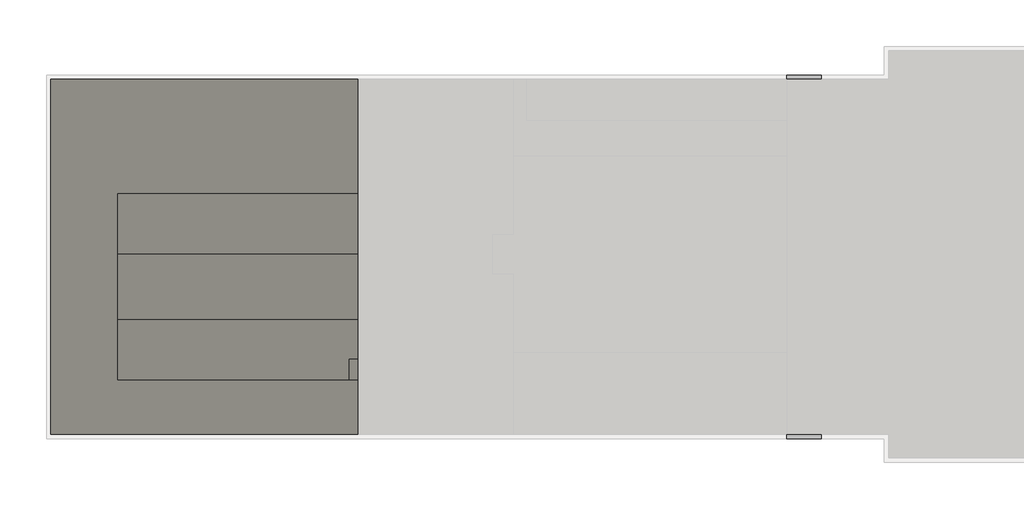
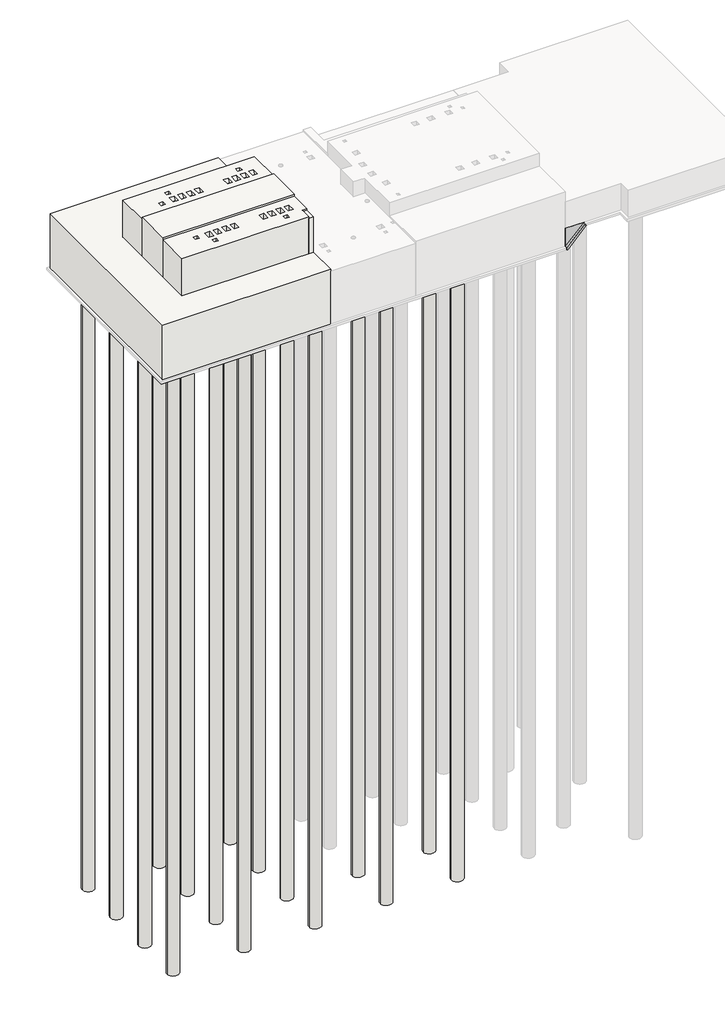
# One storey, part 1 of 2: 20 slabs, 2 proxies.
"""IFC4 building model written with IfcOpenShell, lengths in millimetres."""

from ifc_helpers import new_model, si_unit, point, frame, frame_2d, origin, place, context, project, spatial, polyline, circle_curve, trimmed, segment, composite_curve, outline, extrude, faceted_brep, element, save

model = new_model("IFC4")

# Units and contexts
model_context = context("Model", 3, world=origin())
ifc_project = project(units=[si_unit("LENGTHUNIT", "METRE", prefix="MILLI")], contexts=[model_context])

# Site, building, storey
site = spatial("IfcSite", under=ifc_project)
building = spatial("IfcBuilding", under=site)
storey = spatial("IfcBuildingStorey", under=building, Name="B.O.F", Elevation=2800.0)

# Proxies
placement = place(None, origin())
element("IfcBuildingElementProxy", 1, Name="H_SF_AR_S17_SOG Edge_800x800", ObjectType="H_SF_AR_S17_SOG Edge_800x800", at=placement, inside=storey, context=model_context, shape_type="SweptSolid", body=[
    extrude(outline(polyline([(3600.0, 17000.0), (2800.0, 17000.0), (3600.0, 17800.0), (3600.0, 17000.0)])), frame((0.0, -16046.5096992, 0.0), z_axis=(0.0, 1.0, 0.0), x_axis=(0.0, 0.0, 1.0)), (0.0, 0.0, 1.0), 8200.0),
])
element("IfcBuildingElementProxy", 2, Name="H_SF_AR_S18_Lean_T100_Slab Edge", ObjectType="H_SF_AR_S18_Lean_T100_Slab Edge", at=placement, inside=storey, context=model_context, shape_type="SweptSolid", body=[
    extrude(outline(polyline([(3600.0, 17800.0), (2800.0, 17000.0), (2700.0, 17000.0), (2700.0, 17041.4213562), (3500.0, 17841.4213562), (3500.0, 17800.0), (3600.0, 17800.0)])), frame((0.0, -16146.5096992, 0.0), z_axis=(0.0, 1.0, 0.0), x_axis=(0.0, 0.0, 1.0)), (0.0, 0.0, 1.0), 8400.0),
])

# Slabs
element("IfcSlab", 3, ObjectType="H_SF_AR_B01_EQ FDN_Bitumen_Mat T2440", at=placement, inside=storey, context=model_context, shape_type="Brep", body=[
    faceted_brep([(7095.0, -7846.5096992, 2800.0), (7095.0, -10486.5096992, 2800.0), (1545.0, -10486.5096992, 2800.0), (1545.0, -11886.5096992, 2800.0), (1545.0, -13386.5096992, 2800.0), (1545.0, -14786.5096992, 2800.0), (6895.0, -14786.5096992, 2800.0), (7095.0, -14786.5096992, 2800.0), (7095.0, -16046.5096992, 2800.0), (0.0, -16046.5096992, 2800.0), (0.0, -7846.5096992, 2800.0), (7095.0, -7846.5096992, 5240.0), (0.0, -7846.5096992, 5240.0), (0.0, -16046.5096992, 5240.0), (7095.0, -16046.5096992, 5240.0), (7095.0, -14786.5096992, 5240.0), (1545.0, -14786.5096992, 5240.0), (1545.0, -10486.5096992, 5240.0), (7095.0, -10486.5096992, 5240.0), (7095.0, -7846.5096992, 5150.0), (7095.0, -16046.5096992, 5150.0)], [[[0, 1, 2, 3, 4, 5, 6, 7, 8, 9, 10]], [[11, 12, 13, 14, 15, 16, 17, 18]], [[1, 0, 19, 11, 18]], [[2, 1, 18, 17]], [[5, 4, 3, 2, 17, 16]], [[7, 6, 5, 16, 15]], [[8, 7, 15, 14, 20]], [[9, 8, 20, 14, 13]], [[10, 9, 13, 12]], [[0, 10, 12, 11, 19]]]),
])
element("IfcSlab", 4, ObjectType="H_SF_AR_B01_EQ FDN_Bitumen_Mat T4188", at=placement, inside=storey, context=model_context, shape_type="Brep", body=[
    faceted_brep([(7095.0, -11886.5096992, 2800.0), (7095.0, -13386.5096992, 2800.0), (1545.0, -13386.5096992, 2800.0), (1545.0, -11886.5096992, 2800.0), (7095.0, -13386.5096992, 6988.0), (7095.0, -11886.5096992, 6988.0), (1545.0, -11886.5096992, 6988.0), (1545.0, -13386.5096992, 6988.0), (7095.0, -11886.5096992, 6893.0), (7095.0, -13386.5096992, 6893.0), (1545.0, -13386.5096992, 6893.0), (1545.0, -13386.5096992, 5240.0), (1545.0, -11886.5096992, 6893.0), (1545.0, -11886.5096992, 5240.0)], [[[0, 1, 2, 3]], [[4, 5, 6, 7]], [[1, 0, 8, 5, 4, 9]], [[2, 1, 9, 4, 7, 10, 11]], [[3, 2, 11, 10, 7, 6, 12, 13]], [[0, 3, 13, 12, 6, 5, 8]]]),
])
element("IfcSlab", 5, ObjectType="H_SF_AR_B01_EQ FDN_Bitumen_Mat T4093", at=placement, inside=storey, context=model_context, shape_type="Brep", body=[
    faceted_brep([(6895.0, -14786.5096992, 2800.0), (1545.0, -14786.5096992, 2800.0), (1545.0, -13386.5096992, 2800.0), (7095.0, -13386.5096992, 2800.0), (7095.0, -14316.5096992, 2800.0), (6895.0, -14316.5096992, 2800.0), (1545.0, -14786.5096992, 6893.0), (6895.0, -14786.5096992, 6893.0), (6895.0, -14316.5096992, 6893.0), (7095.0, -14316.5096992, 6893.0), (7095.0, -13386.5096992, 6893.0), (1545.0, -13386.5096992, 6893.0), (2590.0, -13801.5096992, 6893.0), (2760.0, -13801.5096992, 6893.0), (2760.0, -13971.5096992, 6893.0), (2590.0, -13971.5096992, 6893.0), (3110.0, -14286.5096992, 6893.0), (3280.0, -14286.5096992, 6893.0), (3280.0, -14456.5096992, 6893.0), (3110.0, -14456.5096992, 6893.0), (6110.0, -14286.5096992, 6893.0), (6280.0, -14286.5096992, 6893.0), (6280.0, -14456.5096992, 6893.0), (6110.0, -14456.5096992, 6893.0), (3095.0, -14086.5096992, 6893.0), (3095.0, -13786.5096992, 6893.0), (3295.0, -13786.5096992, 6893.0), (3295.0, -14086.5096992, 6893.0), (3445.0, -14086.5096992, 6893.0), (3445.0, -13786.5096992, 6893.0), (3645.0, -13786.5096992, 6893.0), (3645.0, -14086.5096992, 6893.0), (3808.0, -14086.5096992, 6893.0), (3808.0, -13786.5096992, 6893.0), (4008.0, -13786.5096992, 6893.0), (4008.0, -14086.5096992, 6893.0), (4158.0, -14086.5096992, 6893.0), (4158.0, -13786.5096992, 6893.0), (4358.0, -13786.5096992, 6893.0), (4358.0, -14086.5096992, 6893.0), (5382.0, -14086.5096992, 6893.0), (5382.0, -13786.5096992, 6893.0), (5582.0, -13786.5096992, 6893.0), (5582.0, -14086.5096992, 6893.0), (5732.0, -14086.5096992, 6893.0), (5732.0, -13786.5096992, 6893.0), (5932.0, -13786.5096992, 6893.0), (5932.0, -14086.5096992, 6893.0), (6095.0, -14086.5096992, 6893.0), (6095.0, -13786.5096992, 6893.0), (6295.0, -13786.5096992, 6893.0), (6295.0, -14086.5096992, 6893.0), (6445.0, -14086.5096992, 6893.0), (6445.0, -13786.5096992, 6893.0), (6645.0, -13786.5096992, 6893.0), (6645.0, -14086.5096992, 6893.0), (6895.0, -14786.5096992, 5240.0), (6895.0, -14786.5096992, 6833.0), (1545.0, -14786.5096992, 5240.0), (1545.0, -13386.5096992, 5240.0), (7095.0, -14316.5096992, 6833.0), (6895.0, -14316.5096992, 6833.0), (2760.0, -13801.5096992, 6592.9618634), (2590.0, -13801.5096992, 6592.9618634), (2590.0, -13971.5096992, 6592.9618634), (2760.0, -13971.5096992, 6592.9618634), (3280.0, -14286.5096992, 6592.9618634), (3110.0, -14286.5096992, 6592.9618634), (3110.0, -14456.5096992, 6592.9618634), (3280.0, -14456.5096992, 6592.9618634), (6280.0, -14286.5096992, 6592.9618634), (6110.0, -14286.5096992, 6592.9618634), (6110.0, -14456.5096992, 6592.9618634), (6280.0, -14456.5096992, 6592.9618634), (3095.0, -14011.509641, 6138.0), (3295.0, -14011.509641, 6138.0), (3295.0, -13761.5096992, 6138.0), (3095.0, -13761.5096992, 6138.0), (3095.0, -13986.5096992, 6743.0), (3295.0, -13986.5096877, 6743.0), (3445.0, -14011.509641, 6138.0), (3645.0, -14011.509641, 6138.0), (3645.0, -13761.5096992, 6138.0), (3445.0, -13761.5096992, 6138.0), (3445.0, -13986.5096992, 6743.0), (3645.0, -13986.5096877, 6743.0), (3808.0, -14011.509641, 6138.0), (4008.0, -14011.509641, 6138.0), (4008.0, -13761.5096992, 6138.0), (3808.0, -13761.5096992, 6138.0), (3808.0, -13986.5096992, 6743.0), (4008.0, -13986.5096877, 6743.0), (4158.0, -14011.509641, 6138.0), (4358.0, -14011.509641, 6138.0), (4358.0, -13761.5096992, 6138.0), (4158.0, -13761.5096992, 6138.0), (4158.0, -13986.5096992, 6743.0), (4358.0, -13986.5096877, 6743.0), (5382.0, -14011.509641, 6138.0), (5582.0, -14011.509641, 6138.0), (5582.0, -13761.5096992, 6138.0), (5382.0, -13761.5096992, 6138.0), (5382.0, -13986.5096992, 6743.0), (5582.0, -13986.5096877, 6743.0), (5732.0, -14011.509641, 6138.0), (5932.0, -14011.509641, 6138.0), (5932.0, -13761.5096992, 6138.0), (5732.0, -13761.5096992, 6138.0), (5732.0, -13986.5096992, 6743.0), (5932.0, -13986.5096877, 6743.0), (6095.0, -14011.509641, 6138.0), (6295.0, -14011.509641, 6138.0), (6295.0, -13761.5096992, 6138.0), (6095.0, -13761.5096992, 6138.0), (6095.0, -13986.5096992, 6743.0), (6295.0, -13986.5096877, 6743.0), (6445.0, -14011.509641, 6138.0), (6645.0, -14011.509641, 6138.0), (6645.0, -13761.5096992, 6138.0), (6445.0, -13761.5096992, 6138.0), (6445.0, -13986.5096992, 6743.0), (6645.0, -13986.5096877, 6743.0)], [[[0, 1, 2, 3, 4, 5]], [[6, 7, 8, 9, 10, 11], [12, 13, 14, 15], [16, 17, 18, 19], [20, 21, 22, 23], [24, 25, 26, 27], [28, 29, 30, 31], [32, 33, 34, 35], [36, 37, 38, 39], [40, 41, 42, 43], [44, 45, 46, 47], [48, 49, 50, 51], [52, 53, 54, 55]], [[1, 0, 56, 57, 7, 6, 58]], [[2, 1, 58, 6, 11, 59]], [[3, 2, 59, 11, 10]], [[4, 3, 10, 9, 60]], [[5, 4, 60, 9, 8, 61]], [[0, 5, 61, 8, 7, 57, 56]], [[62, 63, 64, 65]], [[63, 62, 13, 12]], [[64, 63, 12, 15]], [[65, 64, 15, 14]], [[62, 65, 14, 13]], [[66, 67, 68, 69]], [[67, 66, 17, 16]], [[68, 67, 16, 19]], [[69, 68, 19, 18]], [[66, 69, 18, 17]], [[70, 71, 72, 73]], [[71, 70, 21, 20]], [[72, 71, 20, 23]], [[73, 72, 23, 22]], [[70, 73, 22, 21]], [[74, 75, 76, 77]], [[74, 77, 25, 24, 78]], [[77, 76, 26, 25]], [[76, 75, 79, 27, 26]], [[75, 74, 78, 79]], [[78, 24, 27, 79]], [[80, 81, 82, 83]], [[80, 83, 29, 28, 84]], [[83, 82, 30, 29]], [[82, 81, 85, 31, 30]], [[81, 80, 84, 85]], [[86, 87, 88, 89]], [[86, 89, 33, 32, 90]], [[89, 88, 34, 33]], [[88, 87, 91, 35, 34]], [[87, 86, 90, 91]], [[92, 93, 94, 95]], [[92, 95, 37, 36, 96]], [[95, 94, 38, 37]], [[94, 93, 97, 39, 38]], [[93, 92, 96, 97]], [[98, 99, 100, 101]], [[98, 101, 41, 40, 102]], [[101, 100, 42, 41]], [[100, 99, 103, 43, 42]], [[99, 98, 102, 103]], [[104, 105, 106, 107]], [[104, 107, 45, 44, 108]], [[107, 106, 46, 45]], [[106, 105, 109, 47, 46]], [[105, 104, 108, 109]], [[110, 111, 112, 113]], [[110, 113, 49, 48, 114]], [[113, 112, 50, 49]], [[112, 111, 115, 51, 50]], [[111, 110, 114, 115]], [[116, 117, 118, 119]], [[116, 119, 53, 52, 120]], [[119, 118, 54, 53]], [[118, 117, 121, 55, 54]], [[117, 116, 120, 121]], [[84, 28, 31, 85]], [[90, 32, 35, 91]], [[96, 36, 39, 97]], [[102, 40, 43, 103]], [[108, 44, 47, 109]], [[114, 48, 51, 115]], [[120, 52, 55, 121]]]),
    faceted_brep([(7095.0, -10486.5096992, 2800.0), (7095.0, -11886.5096992, 2800.0), (1545.0, -11886.5096992, 2800.0), (1545.0, -10486.5096992, 2800.0), (7095.0, -11886.5096992, 6893.0), (7095.0, -10486.5096992, 6893.0), (1545.0, -10486.5096992, 6893.0), (1545.0, -11886.5096992, 6893.0), (2590.0, -11301.5096992, 6893.0), (2760.0, -11301.5096992, 6893.0), (2760.0, -11471.5096992, 6893.0), (2590.0, -11471.5096992, 6893.0), (3110.0, -10816.5096992, 6893.0), (3280.0, -10816.5096992, 6893.0), (3280.0, -10986.5096992, 6893.0), (3110.0, -10986.5096992, 6893.0), (6110.0, -10816.5096992, 6893.0), (6280.0, -10816.5096992, 6893.0), (6280.0, -10986.5096992, 6893.0), (6110.0, -10986.5096992, 6893.0), (3645.0, -11186.5096992, 6893.0), (3645.0, -11486.5096992, 6893.0), (3445.0, -11486.5096992, 6893.0), (3445.0, -11186.5096992, 6893.0), (3295.0, -11186.5096992, 6893.0), (3295.0, -11486.5096992, 6893.0), (3095.0, -11486.5096992, 6893.0), (3095.0, -11186.5096992, 6893.0), (4008.0, -11186.5096992, 6893.0), (4008.0, -11486.5096992, 6893.0), (3808.0, -11486.5096992, 6893.0), (3808.0, -11186.5096992, 6893.0), (4358.0, -11186.5096992, 6893.0), (4358.0, -11486.5096992, 6893.0), (4158.0, -11486.5096992, 6893.0), (4158.0, -11186.5096992, 6893.0), (5582.0, -11186.5096992, 6893.0), (5582.0, -11486.5096992, 6893.0), (5382.0, -11486.5096992, 6893.0), (5382.0, -11186.5096992, 6893.0), (5932.0, -11186.5096992, 6893.0), (5932.0, -11486.5096992, 6893.0), (5732.0, -11486.5096992, 6893.0), (5732.0, -11186.5096992, 6893.0), (6295.0, -11186.5096992, 6893.0), (6295.0, -11486.5096992, 6893.0), (6095.0, -11486.5096992, 6893.0), (6095.0, -11186.5096992, 6893.0), (6645.0, -11186.5096992, 6893.0), (6645.0, -11486.5096992, 6893.0), (6445.0, -11486.5096992, 6893.0), (6445.0, -11186.5096992, 6893.0), (7095.0, -10486.5096992, 5240.0), (1545.0, -11886.5096992, 5240.0), (1545.0, -10486.5096992, 5240.0), (2760.0, -11301.5096992, 6592.9618634), (2590.0, -11301.5096992, 6592.9618634), (2590.0, -11471.5096992, 6592.9618634), (2760.0, -11471.5096992, 6592.9618634), (3280.0, -10816.5096992, 6592.9618634), (3110.0, -10816.5096992, 6592.9618634), (3110.0, -10986.5096992, 6592.9618634), (3280.0, -10986.5096992, 6592.9618634), (6280.0, -10816.5096992, 6592.9618634), (6110.0, -10816.5096992, 6592.9618634), (6110.0, -10986.5096992, 6592.9618634), (6280.0, -10986.5096992, 6592.9618634), (3645.0, -11261.5097575, 6138.0), (3445.0, -11261.5097575, 6138.0), (3445.0, -11511.5096992, 6138.0), (3645.0, -11511.5096992, 6138.0), (3645.0, -11286.5096992, 6743.0), (3445.0, -11286.5097108, 6743.0), (3295.0, -11261.5097575, 6138.0), (3095.0, -11261.5097575, 6138.0), (3095.0, -11511.5096992, 6138.0), (3295.0, -11511.5096992, 6138.0), (3295.0, -11286.5096992, 6743.0), (3095.0, -11286.5097108, 6743.0), (4008.0, -11261.5097575, 6138.0), (3808.0, -11261.5097575, 6138.0), (3808.0, -11511.5096992, 6138.0), (4008.0, -11511.5096992, 6138.0), (4008.0, -11286.5096992, 6743.0), (3808.0, -11286.5097108, 6743.0), (4358.0, -11261.5097575, 6138.0), (4158.0, -11261.5097575, 6138.0), (4158.0, -11511.5096992, 6138.0), (4358.0, -11511.5096992, 6138.0), (4358.0, -11286.5096992, 6743.0), (4158.0, -11286.5097108, 6743.0), (5582.0, -11261.5097575, 6138.0), (5382.0, -11261.5097575, 6138.0), (5382.0, -11511.5096992, 6138.0), (5582.0, -11511.5096992, 6138.0), (5582.0, -11286.5096992, 6743.0), (5382.0, -11286.5097108, 6743.0), (5932.0, -11261.5097575, 6138.0), (5732.0, -11261.5097575, 6138.0), (5732.0, -11511.5096992, 6138.0), (5932.0, -11511.5096992, 6138.0), (5932.0, -11286.5096992, 6743.0), (5732.0, -11286.5097108, 6743.0), (6295.0, -11261.5097575, 6138.0), (6095.0, -11261.5097575, 6138.0), (6095.0, -11511.5096992, 6138.0), (6295.0, -11511.5096992, 6138.0), (6295.0, -11286.5096992, 6743.0), (6095.0, -11286.5097108, 6743.0), (6645.0, -11261.5097575, 6138.0), (6445.0, -11261.5097575, 6138.0), (6445.0, -11511.5096992, 6138.0), (6645.0, -11511.5096992, 6138.0), (6645.0, -11286.5096992, 6743.0), (6445.0, -11286.5097108, 6743.0)], [[[0, 1, 2, 3]], [[4, 5, 6, 7], [8, 9, 10, 11], [12, 13, 14, 15], [16, 17, 18, 19], [20, 21, 22, 23], [24, 25, 26, 27], [28, 29, 30, 31], [32, 33, 34, 35], [36, 37, 38, 39], [40, 41, 42, 43], [44, 45, 46, 47], [48, 49, 50, 51]], [[1, 0, 52, 5, 4]], [[2, 1, 4, 7, 53]], [[3, 2, 53, 7, 6, 54]], [[0, 3, 54, 6, 5, 52]], [[55, 56, 57, 58]], [[59, 60, 61, 62]], [[63, 64, 65, 66]], [[56, 55, 9, 8]], [[57, 56, 8, 11]], [[58, 57, 11, 10]], [[55, 58, 10, 9]], [[60, 59, 13, 12]], [[61, 60, 12, 15]], [[62, 61, 15, 14]], [[59, 62, 14, 13]], [[64, 63, 17, 16]], [[65, 64, 16, 19]], [[66, 65, 19, 18]], [[63, 66, 18, 17]], [[67, 68, 69, 70]], [[67, 70, 21, 20, 71]], [[70, 69, 22, 21]], [[69, 68, 72, 23, 22]], [[68, 67, 71, 72]], [[71, 20, 23, 72]], [[73, 74, 75, 76]], [[73, 76, 25, 24, 77]], [[76, 75, 26, 25]], [[75, 74, 78, 27, 26]], [[74, 73, 77, 78]], [[79, 80, 81, 82]], [[79, 82, 29, 28, 83]], [[82, 81, 30, 29]], [[81, 80, 84, 31, 30]], [[80, 79, 83, 84]], [[85, 86, 87, 88]], [[85, 88, 33, 32, 89]], [[88, 87, 34, 33]], [[87, 86, 90, 35, 34]], [[86, 85, 89, 90]], [[91, 92, 93, 94]], [[91, 94, 37, 36, 95]], [[94, 93, 38, 37]], [[93, 92, 96, 39, 38]], [[92, 91, 95, 96]], [[97, 98, 99, 100]], [[97, 100, 41, 40, 101]], [[100, 99, 42, 41]], [[99, 98, 102, 43, 42]], [[98, 97, 101, 102]], [[103, 104, 105, 106]], [[103, 106, 45, 44, 107]], [[106, 105, 46, 45]], [[105, 104, 108, 47, 46]], [[104, 103, 107, 108]], [[109, 110, 111, 112]], [[109, 112, 49, 48, 113]], [[112, 111, 50, 49]], [[111, 110, 114, 51, 50]], [[110, 109, 113, 114]], [[77, 24, 27, 78]], [[83, 28, 31, 84]], [[89, 32, 35, 90]], [[95, 36, 39, 96]], [[101, 40, 43, 102]], [[107, 44, 47, 108]], [[113, 48, 51, 114]]]),
])
element("IfcSlab", 6, ObjectType="H_SF_AR_B01_EQ FDN_Bitumen_Mat T3493", at=placement, inside=storey, context=model_context, shape_type="Brep", body=[
    faceted_brep([(7095.0, -14316.5096992, 2800.0), (7095.0, -14786.5096992, 2800.0), (6895.0, -14786.5096992, 2800.0), (6895.0, -14316.5096992, 2800.0), (7095.0, -14786.5096992, 6833.0), (7095.0, -14316.5096992, 6833.0), (6895.0, -14316.5096992, 6833.0), (6895.0, -14786.5096992, 6833.0), (7095.0, -14786.5096992, 5240.0), (6895.0, -14786.5096992, 5240.0)], [[[0, 1, 2, 3]], [[4, 5, 6, 7]], [[1, 0, 5, 4, 8]], [[2, 1, 8, 4, 7, 9]], [[3, 2, 9, 7, 6]], [[0, 3, 6, 5]]]),
])
element("IfcSlab", 7, ObjectType="PILE : H_SF_AR_S19_PHC Pile_Hammering_D500_L27.4", at=placement, inside=storey, context=model_context, shape_type="SweptSolid", body=[
    extrude(outline(composite_curve([segment(trimmed(circle_curve(frame_2d((1020.0, -8846.5096992)), 250.0), [point((770.0, -8846.5096992))], [point((1270.0, -8846.5096992))], False, "CARTESIAN"), True, "CONTINUOUS"), segment(trimmed(circle_curve(frame_2d((1020.0, -8846.5096992)), 250.0), [point((1270.0, -8846.5096992))], [point((770.0, -8846.5096992))], False, "CARTESIAN"), True, "CONTINUOUS")], self_intersect=False)), frame((0.0, 0.0, -24600.0), z_axis=(0.0, 0.0, 1.0), x_axis=(1.0, 0.0, 0.0)), (0.0, 0.0, 1.0), 27300.0),
])
element("IfcSlab", 8, ObjectType="PILE : H_SF_AR_S19_PHC Pile_Hammering_D500_L27.4", at=placement, inside=storey, context=model_context, shape_type="SweptSolid", body=[
    extrude(outline(composite_curve([segment(trimmed(circle_curve(frame_2d((4020.0, -8846.5096992)), 250.0), [point((3770.0, -8846.5096992))], [point((4270.0, -8846.5096992))], False, "CARTESIAN"), True, "CONTINUOUS"), segment(trimmed(circle_curve(frame_2d((4020.0, -8846.5096992)), 250.0), [point((4270.0, -8846.5096992))], [point((3770.0, -8846.5096992))], False, "CARTESIAN"), True, "CONTINUOUS")], self_intersect=False)), frame((0.0, 0.0, -24600.0), z_axis=(0.0, 0.0, 1.0), x_axis=(1.0, 0.0, 0.0)), (0.0, 0.0, 1.0), 27300.0),
])
element("IfcSlab", 9, ObjectType="PILE : H_SF_AR_S19_PHC Pile_Hammering_D500_L27.4", at=placement, inside=storey, context=model_context, shape_type="SweptSolid", body=[
    extrude(outline(composite_curve([segment(trimmed(circle_curve(frame_2d((1020.0, -10906.5096992)), 250.0), [point((770.0, -10906.5096992))], [point((1270.0, -10906.5096992))], False, "CARTESIAN"), True, "CONTINUOUS"), segment(trimmed(circle_curve(frame_2d((1020.0, -10906.5096992)), 250.0), [point((1270.0, -10906.5096992))], [point((770.0, -10906.5096992))], False, "CARTESIAN"), True, "CONTINUOUS")], self_intersect=False)), frame((0.0, 0.0, -24600.0), z_axis=(0.0, 0.0, 1.0), x_axis=(1.0, 0.0, 0.0)), (0.0, 0.0, 1.0), 27300.0),
])
element("IfcSlab", 10, ObjectType="PILE : H_SF_AR_S19_PHC Pile_Hammering_D500_L27.4", at=placement, inside=storey, context=model_context, shape_type="SweptSolid", body=[
    extrude(outline(composite_curve([segment(trimmed(circle_curve(frame_2d((4020.0, -10906.5096992)), 250.0), [point((3770.0, -10906.5096992))], [point((4270.0, -10906.5096992))], False, "CARTESIAN"), True, "CONTINUOUS"), segment(trimmed(circle_curve(frame_2d((4020.0, -10906.5096992)), 250.0), [point((4270.0, -10906.5096992))], [point((3770.0, -10906.5096992))], False, "CARTESIAN"), True, "CONTINUOUS")], self_intersect=False)), frame((0.0, 0.0, -24600.0), z_axis=(0.0, 0.0, 1.0), x_axis=(1.0, 0.0, 0.0)), (0.0, 0.0, 1.0), 27300.0),
])
element("IfcSlab", 11, ObjectType="PILE : H_SF_AR_S19_PHC Pile_Hammering_D500_L27.4", at=placement, inside=storey, context=model_context, shape_type="SweptSolid", body=[
    extrude(outline(composite_curve([segment(trimmed(circle_curve(frame_2d((4020.0, -12986.5096992)), 250.0), [point((3770.0, -12986.5096992))], [point((4270.0, -12986.5096992))], False, "CARTESIAN"), True, "CONTINUOUS"), segment(trimmed(circle_curve(frame_2d((4020.0, -12986.5096992)), 250.0), [point((4270.0, -12986.5096992))], [point((3770.0, -12986.5096992))], False, "CARTESIAN"), True, "CONTINUOUS")], self_intersect=False)), frame((0.0, 0.0, -24600.0), z_axis=(0.0, 0.0, 1.0), x_axis=(1.0, 0.0, 0.0)), (0.0, 0.0, 1.0), 27300.0),
])
element("IfcSlab", 12, ObjectType="PILE : H_SF_AR_S19_PHC Pile_Hammering_D500_L27.4", at=placement, inside=storey, context=model_context, shape_type="SweptSolid", body=[
    extrude(outline(composite_curve([segment(trimmed(circle_curve(frame_2d((1020.0, -12986.5096992)), 250.0), [point((770.0, -12986.5096992))], [point((1270.0, -12986.5096992))], False, "CARTESIAN"), True, "CONTINUOUS"), segment(trimmed(circle_curve(frame_2d((1020.0, -12986.5096992)), 250.0), [point((1270.0, -12986.5096992))], [point((770.0, -12986.5096992))], False, "CARTESIAN"), True, "CONTINUOUS")], self_intersect=False)), frame((0.0, 0.0, -24600.0), z_axis=(0.0, 0.0, 1.0), x_axis=(1.0, 0.0, 0.0)), (0.0, 0.0, 1.0), 27300.0),
])
element("IfcSlab", 13, ObjectType="PILE : H_SF_AR_S19_PHC Pile_Hammering_D500_L27.4", at=placement, inside=storey, context=model_context, shape_type="SweptSolid", body=[
    extrude(outline(composite_curve([segment(trimmed(circle_curve(frame_2d((1020.0, -15046.5096992)), 250.0), [point((770.0, -15046.5096992))], [point((1270.0, -15046.5096992))], False, "CARTESIAN"), True, "CONTINUOUS"), segment(trimmed(circle_curve(frame_2d((1020.0, -15046.5096992)), 250.0), [point((1270.0, -15046.5096992))], [point((770.0, -15046.5096992))], False, "CARTESIAN"), True, "CONTINUOUS")], self_intersect=False)), frame((0.0, 0.0, -24600.0), z_axis=(0.0, 0.0, 1.0), x_axis=(1.0, 0.0, 0.0)), (0.0, 0.0, 1.0), 27300.0),
])
element("IfcSlab", 14, ObjectType="PILE : H_SF_AR_S19_PHC Pile_Hammering_D500_L27.4", at=placement, inside=storey, context=model_context, shape_type="SweptSolid", body=[
    extrude(outline(composite_curve([segment(trimmed(circle_curve(frame_2d((4020.0, -15046.5096992)), 250.0), [point((3770.0, -15046.5096992))], [point((4270.0, -15046.5096992))], False, "CARTESIAN"), True, "CONTINUOUS"), segment(trimmed(circle_curve(frame_2d((4020.0, -15046.5096992)), 250.0), [point((4270.0, -15046.5096992))], [point((3770.0, -15046.5096992))], False, "CARTESIAN"), True, "CONTINUOUS")], self_intersect=False)), frame((0.0, 0.0, -24600.0), z_axis=(0.0, 0.0, 1.0), x_axis=(1.0, 0.0, 0.0)), (0.0, 0.0, 1.0), 27300.0),
])
element("IfcSlab", 15, ObjectType="PILE : H_SF_AR_S19_PHC Pile_Hammering_D500_L27.4", at=placement, inside=storey, context=model_context, shape_type="SweptSolid", body=[
    extrude(outline(composite_curve([segment(trimmed(circle_curve(frame_2d((7020.0, -8846.5096992)), 250.0), [point((6770.0, -8846.5096992))], [point((7270.0, -8846.5096992))], False, "CARTESIAN"), True, "CONTINUOUS"), segment(trimmed(circle_curve(frame_2d((7020.0, -8846.5096992)), 250.0), [point((7270.0, -8846.5096992))], [point((6770.0, -8846.5096992))], False, "CARTESIAN"), True, "CONTINUOUS")], self_intersect=False)), frame((0.0, 0.0, -24600.0), z_axis=(0.0, 0.0, 1.0), x_axis=(1.0, 0.0, 0.0)), (0.0, 0.0, 1.0), 27300.0),
])
element("IfcSlab", 16, ObjectType="PILE : H_SF_AR_S19_PHC Pile_Hammering_D500_L27.4", at=placement, inside=storey, context=model_context, shape_type="SweptSolid", body=[
    extrude(outline(composite_curve([segment(trimmed(circle_curve(frame_2d((7020.0, -10906.5096992)), 250.0), [point((6770.0, -10906.5096992))], [point((7270.0, -10906.5096992))], False, "CARTESIAN"), True, "CONTINUOUS"), segment(trimmed(circle_curve(frame_2d((7020.0, -10906.5096992)), 250.0), [point((7270.0, -10906.5096992))], [point((6770.0, -10906.5096992))], False, "CARTESIAN"), True, "CONTINUOUS")], self_intersect=False)), frame((0.0, 0.0, -24600.0), z_axis=(0.0, 0.0, 1.0), x_axis=(1.0, 0.0, 0.0)), (0.0, 0.0, 1.0), 27300.0),
])
element("IfcSlab", 17, ObjectType="PILE : H_SF_AR_S19_PHC Pile_Hammering_D500_L27.4", at=placement, inside=storey, context=model_context, shape_type="SweptSolid", body=[
    extrude(outline(composite_curve([segment(trimmed(circle_curve(frame_2d((7020.0, -12986.5096992)), 250.0), [point((6770.0, -12986.5096992))], [point((7270.0, -12986.5096992))], False, "CARTESIAN"), True, "CONTINUOUS"), segment(trimmed(circle_curve(frame_2d((7020.0, -12986.5096992)), 250.0), [point((7270.0, -12986.5096992))], [point((6770.0, -12986.5096992))], False, "CARTESIAN"), True, "CONTINUOUS")], self_intersect=False)), frame((0.0, 0.0, -24600.0), z_axis=(0.0, 0.0, 1.0), x_axis=(1.0, 0.0, 0.0)), (0.0, 0.0, 1.0), 27300.0),
])
element("IfcSlab", 18, ObjectType="PILE : H_SF_AR_S19_PHC Pile_Hammering_D500_L27.4", at=placement, inside=storey, context=model_context, shape_type="SweptSolid", body=[
    extrude(outline(composite_curve([segment(trimmed(circle_curve(frame_2d((7020.0, -15046.5096992)), 250.0), [point((6770.0, -15046.5096992))], [point((7270.0, -15046.5096992))], False, "CARTESIAN"), True, "CONTINUOUS"), segment(trimmed(circle_curve(frame_2d((7020.0, -15046.5096992)), 250.0), [point((7270.0, -15046.5096992))], [point((6770.0, -15046.5096992))], False, "CARTESIAN"), True, "CONTINUOUS")], self_intersect=False)), frame((0.0, 0.0, -24600.0), z_axis=(0.0, 0.0, 1.0), x_axis=(1.0, 0.0, 0.0)), (0.0, 0.0, 1.0), 27300.0),
])
element("IfcSlab", 19, ObjectType="PILE : H_SF_AR_S19_PHC Pile_Hammering_D500_L27.4", at=placement, inside=storey, context=model_context, shape_type="SweptSolid", body=[
    extrude(outline(composite_curve([segment(trimmed(circle_curve(frame_2d((10020.0, -12986.5096992)), 250.0), [point((9770.0, -12986.5096992))], [point((10270.0, -12986.5096992))], False, "CARTESIAN"), True, "CONTINUOUS"), segment(trimmed(circle_curve(frame_2d((10020.0, -12986.5096992)), 250.0), [point((10270.0, -12986.5096992))], [point((9770.0, -12986.5096992))], False, "CARTESIAN"), True, "CONTINUOUS")], self_intersect=False)), frame((0.0, 0.0, -24600.0), z_axis=(0.0, 0.0, 1.0), x_axis=(1.0, 0.0, 0.0)), (0.0, 0.0, 1.0), 27300.0),
])
element("IfcSlab", 20, ObjectType="PILE : H_SF_AR_S19_PHC Pile_Hammering_D500_L27.4", at=placement, inside=storey, context=model_context, shape_type="SweptSolid", body=[
    extrude(outline(composite_curve([segment(trimmed(circle_curve(frame_2d((10020.0, -15046.5096992)), 250.0), [point((9770.0, -15046.5096992))], [point((10270.0, -15046.5096992))], False, "CARTESIAN"), True, "CONTINUOUS"), segment(trimmed(circle_curve(frame_2d((10020.0, -15046.5096992)), 250.0), [point((10270.0, -15046.5096992))], [point((9770.0, -15046.5096992))], False, "CARTESIAN"), True, "CONTINUOUS")], self_intersect=False)), frame((0.0, 0.0, -24600.0), z_axis=(0.0, 0.0, 1.0), x_axis=(1.0, 0.0, 0.0)), (0.0, 0.0, 1.0), 27300.0),
])
element("IfcSlab", 21, ObjectType="PILE : H_SF_AR_S19_PHC Pile_Hammering_D500_L27.4", at=placement, inside=storey, context=model_context, shape_type="SweptSolid", body=[
    extrude(outline(composite_curve([segment(trimmed(circle_curve(frame_2d((13020.0, -15046.5096992)), 250.0), [point((12770.0, -15046.5096992))], [point((13270.0, -15046.5096992))], False, "CARTESIAN"), True, "CONTINUOUS"), segment(trimmed(circle_curve(frame_2d((13020.0, -15046.5096992)), 250.0), [point((13270.0, -15046.5096992))], [point((12770.0, -15046.5096992))], False, "CARTESIAN"), True, "CONTINUOUS")], self_intersect=False)), frame((0.0, 0.0, -24600.0), z_axis=(0.0, 0.0, 1.0), x_axis=(1.0, 0.0, 0.0)), (0.0, 0.0, 1.0), 27300.0),
])
element("IfcSlab", 22, ObjectType="PILE : H_SF_AR_S19_PHC Pile_Hammering_D500_L27.4", at=placement, inside=storey, context=model_context, shape_type="SweptSolid", body=[
    extrude(outline(composite_curve([segment(trimmed(circle_curve(frame_2d((13020.0, -12986.5096992)), 250.0), [point((12770.0, -12986.5096992))], [point((13270.0, -12986.5096992))], False, "CARTESIAN"), True, "CONTINUOUS"), segment(trimmed(circle_curve(frame_2d((13020.0, -12986.5096992)), 250.0), [point((13270.0, -12986.5096992))], [point((12770.0, -12986.5096992))], False, "CARTESIAN"), True, "CONTINUOUS")], self_intersect=False)), frame((0.0, 0.0, -24600.0), z_axis=(0.0, 0.0, 1.0), x_axis=(1.0, 0.0, 0.0)), (0.0, 0.0, 1.0), 27300.0),
])

save(model, "model.ifc")

# Revit data of these elements
# Project information
#   H_Seismic Condition = "A as per ASCE 7-10"
#   H_Soil Condition = "C as per ASCE 7-10"
#   H_Basic Wind Speed = "58.3m/s ASCE7-10"
#   Building Name = "FUEL GAS SUPPLY SYSTEM SHELTER"
#   H_DS Project Code = "FAASA2302"
#   H_Project Abbreviation = "SACE2"
#   H_Project Division = "화공"
#   H_Project Finish = "2027-03-05"
#   H_Project Location = "Jafurah, Saudi Arabia"
#   H_Project Start = "2024-01-03"
#   H_Project Type = "EPC"
#   H_Smart Code = "FAASA2302"
#   Project Issue Date = "Issue Date"
#   Project Status = "Project Status"
#   Client Name = "Owner"
#   Project Address = "Enter address here"
#   Project Name = "Project Name"
#   Project Number = "0001"
#   RoomBookInternationalBuildNumber = "ZgA=BAAAAA==2023BgFlAAAAAQQAAAABAQAAAAYBZAAAAAHnBwAABAQAAAABTwQAAAcH1"
# Grids (mm)
#   "3": line (24520, 2752.995) -> (24520, -21557.759)
#   "A": line (-3097.566, -7186.51) -> (27348.139, -7186.51)
#   "E": line (-3097.566, -16586.51) -> (27348.139, -16586.51)
#   "C": line (-3097.566, -14136.51) -> (27348.139, -14136.51)
#   "6": line (1020, 2752.995) -> (1020, -21557.759)
#   "5": line (8020, 2752.995) -> (8020, -21557.759)
#   "B": line (-3097.566, -7846.51) -> (27348.139, -7846.51)
#   "J": line (-3097.566, -12636.51) -> (27348.139, -12636.51)
#   "K": line (4870, 2752.995) -> (4870, -21557.759)
#   "4": line (16020, 2752.995) -> (16020, -21557.759)
#   "D": line (-3097.566, -16046.51) -> (27348.139, -16046.51)
# Type "H_SF_AR_B01_EQ FDN_Bitumen_Mat T2440"
#   Type Comments = "구조_콘크리트"
#   Type Mark = "MF00"
#   Layers, outside or top first: 2440 mm "Concrete_f'c=24MPa(Cylender)" (function 1)
# Type "H_SF_AR_B01_EQ FDN_Bitumen_Mat T4188"
#   Type Comments = "CV-AG"
#   Description = "AG Equipment Foundation"
#   Type Mark = "MF00"
#   Layers, outside or top first: 4188 mm "Concrete_f'c=24MPa(Cylender)" (function 1)
# Type "H_SF_AR_B01_EQ FDN_Bitumen_Mat T4093"
#   Type Comments = "구조_콘크리트"
#   Type Mark = "MF00"
#   Layers, outside or top first: 4093 mm "Concrete_f'c=24MPa(Cylender)" (function 1)
# Type "H_SF_AR_B01_EQ FDN_Bitumen_Mat T3493"
#   Type Comments = "구조_콘크리트"
#   Type Mark = "MF00"
#   Layers, outside or top first: 4033 mm "Concrete_f'c=24MPa(Cylender)" (function 1)
# Type "PILE : H_SF_AR_S19_PHC Pile_Hammering_D500_L27.4"
#   Type Comments = "CV-UG"
#   Assembly Code = "A1020120"
#   반지름 = 250 mm
#   최소 내포 = 100 mm
#   Diameter = 500 mm
#   Depth = 27400 mm
#   Structural Material [instance default] = none
# Element 1 (IfcBuildingElementProxy, "H_SF_AR_S17_SOG Edge_800x800")
#   Phase Created = New Construction
#   Materials on its faces: "Concrete_f'c=24MPa(Cylender)"
# Element 2 (IfcBuildingElementProxy, "H_SF_AR_S18_Lean_T100_Slab Edge")
#   Phase Created = New Construction
#   Materials on its faces: "Concrete_Lean_f'c=14MPa(Cylender)"
# Element 3 (IfcSlab, "H_SF_AR_B01_EQ FDN_Bitumen_Mat T2440")
#   Comments = ""
#   Height Offset From Level = 2440 mm
#   built-in parameter 1001954 = 1
#   Phase Created = New Construction
#   Materials on its faces: "Concrete_f'c=24MPa(Cylender)"
# Element 4 (IfcSlab, "H_SF_AR_B01_EQ FDN_Bitumen_Mat T4188")
#   Comments = ""
#   Height Offset From Level = 4188 mm
#   built-in parameter 1001954 = 1
#   Phase Created = New Construction
#   Materials on its faces: "Concrete_f'c=24MPa(Cylender)"
# Element 5 (IfcSlab, "H_SF_AR_B01_EQ FDN_Bitumen_Mat T4093")
#   Comments = ""
#   Height Offset From Level = 4093 mm
#   built-in parameter 1001954 = 1
#   Phase Created = New Construction
#   Materials on its faces: "Concrete_f'c=24MPa(Cylender)"
# Element 6 (IfcSlab, "H_SF_AR_B01_EQ FDN_Bitumen_Mat T3493")
#   Comments = ""
#   Height Offset From Level = 4033 mm
#   built-in parameter 1001954 = 1
#   Phase Created = New Construction
#   Materials on its faces: "Concrete_f'c=24MPa(Cylender)"
# Element 7 (IfcSlab, "PILE : H_SF_AR_S19_PHC Pile_Hammering_D500_L27.4")
#   Mark = "001"
#   Structural Material = Concrete_f'c=28MPa(Cylender)
#   Phase Created = New Construction
#   Materials on its faces: "Concrete_f'c=28MPa(Cylender)"
# Element 8 (IfcSlab, "PILE : H_SF_AR_S19_PHC Pile_Hammering_D500_L27.4")
#   Mark = "005"
#   Structural Material = Concrete_f'c=28MPa(Cylender)
#   Phase Created = New Construction
#   Materials on its faces: "Concrete_f'c=28MPa(Cylender)"
# Element 9 (IfcSlab, "PILE : H_SF_AR_S19_PHC Pile_Hammering_D500_L27.4")
#   Mark = "002"
#   Structural Material = Concrete_f'c=28MPa(Cylender)
#   Phase Created = New Construction
#   Materials on its faces: "Concrete_f'c=28MPa(Cylender)"
# Element 10 (IfcSlab, "PILE : H_SF_AR_S19_PHC Pile_Hammering_D500_L27.4")
#   Mark = "006"
#   Structural Material = Concrete_f'c=28MPa(Cylender)
#   Phase Created = New Construction
#   Materials on its faces: "Concrete_f'c=28MPa(Cylender)"
# Element 11 (IfcSlab, "PILE : H_SF_AR_S19_PHC Pile_Hammering_D500_L27.4")
#   Mark = "007"
#   Structural Material = Concrete_f'c=28MPa(Cylender)
#   Phase Created = New Construction
#   Materials on its faces: "Concrete_f'c=28MPa(Cylender)"
# Element 12 (IfcSlab, "PILE : H_SF_AR_S19_PHC Pile_Hammering_D500_L27.4")
#   Mark = "003"
#   Structural Material = Concrete_f'c=28MPa(Cylender)
#   Phase Created = New Construction
#   Materials on its faces: "Concrete_f'c=28MPa(Cylender)"
# Element 13 (IfcSlab, "PILE : H_SF_AR_S19_PHC Pile_Hammering_D500_L27.4")
#   Mark = "004"
#   Structural Material = Concrete_f'c=28MPa(Cylender)
#   Phase Created = New Construction
#   Materials on its faces: "Concrete_f'c=28MPa(Cylender)"
# Element 14 (IfcSlab, "PILE : H_SF_AR_S19_PHC Pile_Hammering_D500_L27.4")
#   Mark = "008"
#   Structural Material = Concrete_f'c=28MPa(Cylender)
#   Phase Created = New Construction
#   Materials on its faces: "Concrete_f'c=28MPa(Cylender)"
# Element 15 (IfcSlab, "PILE : H_SF_AR_S19_PHC Pile_Hammering_D500_L27.4")
#   Mark = "009"
#   Structural Material = Concrete_f'c=28MPa(Cylender)
#   Phase Created = New Construction
#   Materials on its faces: "Concrete_f'c=28MPa(Cylender)"
# Element 16 (IfcSlab, "PILE : H_SF_AR_S19_PHC Pile_Hammering_D500_L27.4")
#   Mark = "010"
#   Structural Material = Concrete_f'c=28MPa(Cylender)
#   Phase Created = New Construction
#   Materials on its faces: "Concrete_f'c=28MPa(Cylender)"
# Element 17 (IfcSlab, "PILE : H_SF_AR_S19_PHC Pile_Hammering_D500_L27.4")
#   Mark = "011"
#   Structural Material = Concrete_f'c=28MPa(Cylender)
#   Phase Created = New Construction
#   Materials on its faces: "Concrete_f'c=28MPa(Cylender)"
# Element 18 (IfcSlab, "PILE : H_SF_AR_S19_PHC Pile_Hammering_D500_L27.4")
#   Mark = "012"
#   Structural Material = Concrete_f'c=28MPa(Cylender)
#   Phase Created = New Construction
#   Materials on its faces: "Concrete_f'c=28MPa(Cylender)"
# Element 19 (IfcSlab, "PILE : H_SF_AR_S19_PHC Pile_Hammering_D500_L27.4")
#   Mark = "015"
#   Structural Material = Concrete_f'c=28MPa(Cylender)
#   Phase Created = New Construction
#   Materials on its faces: "Concrete_f'c=28MPa(Cylender)"
# Element 20 (IfcSlab, "PILE : H_SF_AR_S19_PHC Pile_Hammering_D500_L27.4")
#   Mark = "016"
#   Structural Material = Concrete_f'c=28MPa(Cylender)
#   Phase Created = New Construction
#   Materials on its faces: "Concrete_f'c=28MPa(Cylender)"
# Element 21 (IfcSlab, "PILE : H_SF_AR_S19_PHC Pile_Hammering_D500_L27.4")
#   Mark = "020"
#   Structural Material = Concrete_f'c=28MPa(Cylender)
#   Phase Created = New Construction
#   Materials on its faces: "Concrete_f'c=28MPa(Cylender)"
# Element 22 (IfcSlab, "PILE : H_SF_AR_S19_PHC Pile_Hammering_D500_L27.4")
#   Mark = "019"
#   Structural Material = Concrete_f'c=28MPa(Cylender)
#   Phase Created = New Construction
#   Materials on its faces: "Concrete_f'c=28MPa(Cylender)"
# Materials
#   "Concrete_f'c=24MPa(Cylender)": class "Concrete", colour RGB 176 176 176, transparency 0, Description = "EPOXY PAINT\rON STEEL TROWEL FINISH", Cost = 0, Image = Concrete.Cast-In-Place.Flat.Polished.Grey.jpg
#   "Concrete_Lean_f'c=14MPa(Cylender)": class "Concrete", colour RGB 177 177 177, transparency 0, Description = "Reinf. Conc.", Cost = 0
#   "Concrete_f'c=28MPa(Cylender)": class "Concrete", colour RGB 176 176 176, transparency 0, Description = "Reinf. Conc.", Cost = 0, Image = Concrete.Cast-In-Place.Flat.Polished.Grey.jpg
